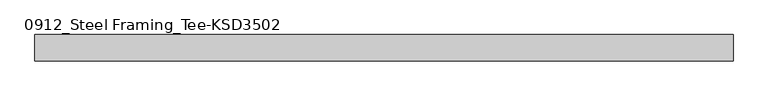
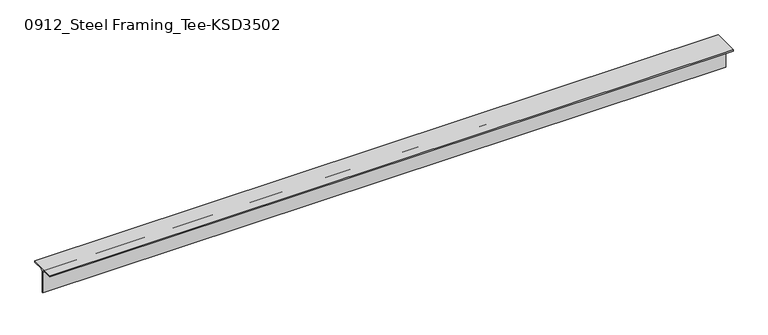
"""IFC4 building model written with IfcOpenShell, lengths in millimetres: member geometry, 0912_Steel Framing_Tee-KSD3502 : H_SB_ASB_CT-150x150x6.5x9."""

from ifc_helpers import new_model, si_unit, point, frame, frame_2d, origin, place, context, project, spatial, polyline, circle_curve, trimmed, segment, composite_curve, outline, extrude, source, transform, mapped, element, save


def member_0912_steel_framing_tee_ksd3502_60f01093(model_context):
    return source(origin(), model_context, "Body", "SweptSolid", [
        extrude(outline(composite_curve([segment(polyline([(-75.0, 75.0), (75.0, 75.0), (75.0, 66.0), (16.25, 66.0)]), True, "CONTINUOUS"), segment(trimmed(circle_curve(frame_2d((16.25, 53.0)), 13.0), [point((16.25, 66.0))], [point((3.25, 53.0))], True, "CARTESIAN"), True, "CONTINUOUS"), segment(polyline([(3.25, 53.0), (3.25, -75.0), (-3.25, -75.0), (-3.25, 53.0)]), True, "CONTINUOUS"), segment(trimmed(circle_curve(frame_2d((-16.25, 53.0)), 13.0), [point((-3.25, 53.0))], [point((-16.25, 66.0))], True, "CARTESIAN"), True, "CONTINUOUS"), segment(polyline([(-16.25, 66.0), (-75.0, 66.0), (-75.0, 75.0)]), True, "CONTINUOUS")], self_intersect=False)), frame((-1975.65, 0.0, 0.0), z_axis=(1.0, 0.0, 0.0), x_axis=(0.0, 1.0, 0.0)), (0.0, 0.0, 1.0), 3955.0),
    ])


if __name__ == "__main__":
    model = new_model("IFC4")
    model_context = context("Model", 3, world=origin())
    ifc_project = project(units=[si_unit("LENGTHUNIT", "METRE", prefix="MILLI")], contexts=[model_context])
    site = spatial("IfcSite", under=ifc_project)
    building = spatial("IfcBuilding", under=site)
    placement = place(None, origin())
    member_0912_steel_framing_tee_ksd3502_shape = member_0912_steel_framing_tee_ksd3502_60f01093(model_context)
    element("IfcMember", 1, ObjectType="0912_Steel Framing_Tee-KSD3502 : H_SB_ASB_CT-150x150x6.5x9", at=placement, inside=building, context=model_context, shape_type="MappedRepresentation", body=[
        mapped(member_0912_steel_framing_tee_ksd3502_shape, transform((0.0, 0.0, 0.0), x_axis=(1.0, 0.0, 0.0), y_axis=(0.0, 1.0, 0.0), z_axis=(0.0, 0.0, 1.0))),
    ])
    save(model, "model.ifc")

# Revit data of these elements
# Type "0912_Steel Framing_Tee-KSD3502 : H_SB_ASB_CT-150x150x6.5x9"
#   H_WM Code_1 = "S01AA003-00001 | Main Steel Structure Fabrication Work | Shelter/Building | Light Steel - Standard (30KG/M>Weight) | Material: (   )"
#   H_WM Code_2 = "S03AA029-00001 | Main Steel Structure Erection Work | Shelter/Building | Light Steel (30KG/M>Weight) | Material: (   )"
#   H_WM Code_3 = "S01AA010-00001 | Main Steel Structure Fabrication Work | Shelter/Building | Steel Painting/Coating | for Non-Fireproofed Steel Surface, Surface Preparation, Primer, Second & Final Coat | Material: (   )"
#   H_Q'ty Cal Type Tag = "SB-Q2"
#   Width = 15.0 cm
#   Web Thickness = 0.65 cm
#   Web Fillet = 1.3 cm
#   Section Area = 23.39 cm²
#   Perimeter = 0.60 m²/m
#   Nominal Weight = 18.40 kgf/m
#   Height = 15.0 cm
#   Flange Thickness = 0.9 cm
#   Centroid Vertical = 7.5 cm
#   Centroid Horizontal = 7.5 cm
#   Length [instance default] = 1.5000 m
#   Structural Material [instance default] = Steel, 45-345
#   Warping Constant = (empty or 0)
#   Torsional Moment of Inertia = 0
#   Section Name Key = ""
#   Plastic Modulus weak axis = 0
#   Plastic Modulus strong axis = 0
#   Moment of Inertia weak axis = 0
#   Moment of Inertia strong axis = 0
#   Elastic Modulus weak axis = 0
#   Elastic Modulus strong axis = 0
#   Bolt Spacing = 0
#   Assembly Code = ""
# Element 1 (IfcMember, "0912_Steel Framing_Tee-KSD3502 : H_SB_ASB_CT-150x150x6.5x9")
#   Structural Material = none
# Materials
#   "Steel, 45-345": class "Metal", colour RGB 189 187 185, transparency 0, Description = "Steel 345 MPa", Cost = 0
